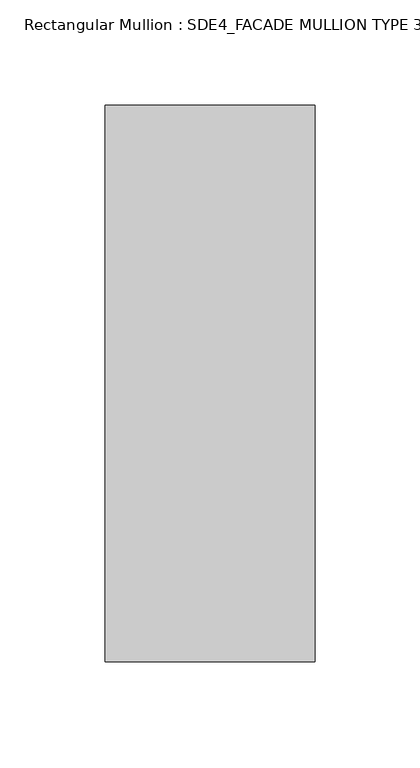
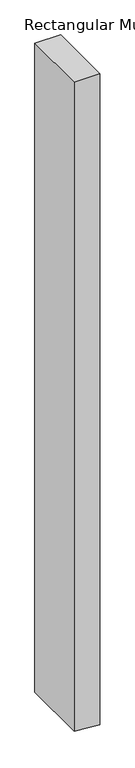
"""IFC4 building model written with IfcOpenShell, lengths in millimetres: member geometry, Rectangular Mullion : SDE4_FACADE MULLION TYPE 3."""

from ifc_helpers import new_model, si_unit, frame, origin, place, context, project, spatial, polyline, outline, extrude, source, transform, mapped, element, save


def rectangular_mullion_sde4_facade_mullion_type_3_804b621b(model_context):
    return source(origin(), model_context, "Body", "SweptSolid", [
        extrude(outline(polyline([(0.0, 50.0), (0.0, -50.0), (-2671.3042242, -50.0), (-2675.3703033, 3.056508), (-2678.9679006, 50.0), (0.0, 50.0)])), frame((0.0, -132.5, 0.0), z_axis=(0.0, 1.0, 0.0), x_axis=(0.0, 0.0, 1.0)), (0.0, 0.0, 1.0), 265.0),
    ])


if __name__ == "__main__":
    model = new_model("IFC4")
    model_context = context("Model", 3, world=origin())
    ifc_project = project(units=[si_unit("LENGTHUNIT", "METRE", prefix="MILLI")], contexts=[model_context])
    site = spatial("IfcSite", under=ifc_project)
    building = spatial("IfcBuilding", under=site)
    placement = place(None, origin())
    rectangular_mullion_sde4_facade_mullion_type_3_shape = rectangular_mullion_sde4_facade_mullion_type_3_804b621b(model_context)
    element("IfcMember", 1, ObjectType="Rectangular Mullion : SDE4_FACADE MULLION TYPE 3", at=placement, inside=building, context=model_context, shape_type="MappedRepresentation", body=[
        mapped(rectangular_mullion_sde4_facade_mullion_type_3_shape, transform((0.0, 0.0, 0.0), x_axis=(1.0, 0.0, 0.0), y_axis=(0.0, 1.0, 0.0), z_axis=(0.0, 0.0, 1.0))),
    ])
    save(model, "model.ifc")

# Revit data of these elements
# Type "Rectangular Mullion : SDE4_FACADE MULLION TYPE 3"
#   built-in parameter 1007322 = 0.869423 (stored number, unit not read)
#   built-in parameter 1007321 = 0.164042 (stored number, unit not read)
#   built-in parameter 1007320 = 0.164042 (stored number, unit not read)
